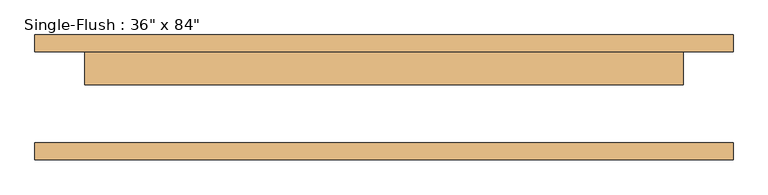
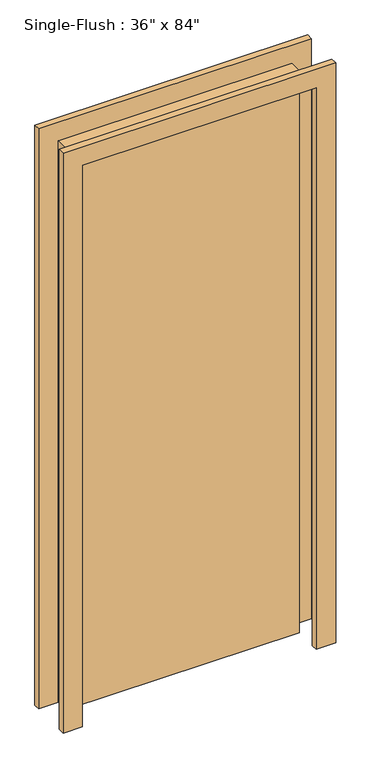
"""IFC4 building model written with IfcOpenShell, lengths in millimetres: door geometry."""

import ifcopenshell
import ifcopenshell.guid

model = None  # the IFC model being written
_history = None  # IfcOwnerHistory: only IFC2X3 demands one
_inside = {}  # id of a spatial element -> (the spatial element, [elements in it])
_under = {}  # id of a project, library or spatial element -> (it, [spatial elements below it])
_declared = {}  # id of a project -> (the project, [libraries it declares])
_typed = {}  # id of a type object -> (the type object, [elements of that type])
_made_of = {}  # id of a material, layer set ... -> (it, [elements and type objects made of it])


def new_model(schema):
    """Start an empty IFC model of exactly this schema.

    Asked for "IFC4X3", IfcOpenShell would pick the latest addendum, in which some entities
    have other attributes; the version numbers below select the first issue.
    IFC2X3 requires an IfcOwnerHistory on every rooted entity: one is made here for all.
    """
    global model, _history
    if schema == "IFC4X3":
        model = ifcopenshell.file(schema_version=(4, 3, 0, 0))
    else:
        model = ifcopenshell.file(schema=schema)
    _inside.clear()
    _under.clear()
    _declared.clear()
    _typed.clear()
    _made_of.clear()
    _history = None
    if model.schema == "IFC2X3":
        org = make("IfcOrganization", Name="unknown")
        user = make(
            "IfcPersonAndOrganization",
            ThePerson=make("IfcPerson", FamilyName="unknown"),
            TheOrganization=org,
        )
        app = make(
            "IfcApplication",
            ApplicationDeveloper=org,
            Version="unknown",
            ApplicationFullName="unknown",
            ApplicationIdentifier="unknown",
        )
        _history = make(
            "IfcOwnerHistory",
            OwningUser=user,
            OwningApplication=app,
            ChangeAction="ADDED",
            CreationDate=0,
        )
    return model


def make(cls, **values):
    """One entity of the class cls with the attributes given. An attribute that is None is left unset."""
    return model.create_entity(
        cls, **{name: value for name, value in values.items() if value is not None}
    )


def rooted(cls, **values):
    """An entity with a GlobalId (a new one), such as an element, a storey or a relation."""
    return make(cls, GlobalId=ifcopenshell.guid.new(), OwnerHistory=_history, **values)


def si_unit(unit_type, name, prefix=None):
    """IfcSIUnit, for example si_unit("LENGTHUNIT", "METRE", prefix="MILLI")."""
    return make("IfcSIUnit", UnitType=unit_type, Prefix=prefix, Name=name)


def assignment(units):
    """IfcUnitAssignment: the units of a project."""
    return None if units is None else make("IfcUnitAssignment", Units=units)


def point(xyz):
    """IfcCartesianPoint."""
    return None if xyz is None else make("IfcCartesianPoint", Coordinates=xyz)


def direction(xyz):
    """IfcDirection."""
    return None if xyz is None else make("IfcDirection", DirectionRatios=xyz)


def frame(location, z_axis=None, x_axis=None):
    """IfcAxis2Placement3D, a coordinate frame: its origin and axes. An axis left out is left unset."""
    return make(
        "IfcAxis2Placement3D",
        Location=point(location),
        Axis=direction(z_axis),
        RefDirection=direction(x_axis),
    )


def origin():
    """The frame at (0, 0, 0) with its axes left unset."""
    return frame((0.0, 0.0, 0.0))


def origin_with_axes():
    """The frame at (0, 0, 0) with the z axis (0, 0, 1) and the x axis (1, 0, 0) written out."""
    return frame((0.0, 0.0, 0.0), z_axis=(0.0, 0.0, 1.0), x_axis=(1.0, 0.0, 0.0))


def place(relative_to, where):
    """IfcLocalPlacement: puts the frame where relative to a parent placement (None: the world)."""
    return make(
        "IfcLocalPlacement", PlacementRelTo=relative_to, RelativePlacement=where
    )


def context(
    kind, dimensions, precision=None, world=None, true_north=None, identifier=None
):
    """IfcGeometricRepresentationContext, for example the 3D "Model" context."""
    return make(
        "IfcGeometricRepresentationContext",
        ContextIdentifier=identifier,
        ContextType=kind,
        CoordinateSpaceDimension=dimensions,
        Precision=precision,
        WorldCoordinateSystem=world,
        TrueNorth=true_north,
    )


def project(units=None, contexts=None):
    """IfcProject with its units and contexts."""
    return rooted(
        "IfcProject",
        Name="project",
        RepresentationContexts=contexts,
        UnitsInContext=assignment(units),
    )


def spatial(cls, under=None, at=None, **own):
    """A site, building, storey or space (cls), placed at a placement, below another one or the project."""
    s = rooted(cls, ObjectPlacement=at, **own)
    if under is not None:
        _under.setdefault(under.id(), (under, []))[1].append(s)
    return s


def polyline(points):
    """IfcPolyline through the points."""
    return make("IfcPolyline", Points=[point(p) for p in points])


def outline(outer, holes=None, kind="AREA"):
    """IfcArbitraryClosedProfileDef: a profile drawn as a closed curve; with holes, ...WithVoids."""
    if holes is None:
        return make("IfcArbitraryClosedProfileDef", ProfileType=kind, OuterCurve=outer)
    return make(
        "IfcArbitraryProfileDefWithVoids",
        ProfileType=kind,
        OuterCurve=outer,
        InnerCurves=holes,
    )


def extrude(swept, where, along, depth):
    """IfcExtrudedAreaSolid: the profile swept, set in the frame where, extruded along a direction by depth."""
    return make(
        "IfcExtrudedAreaSolid",
        SweptArea=swept,
        Position=where,
        ExtrudedDirection=direction(along),
        Depth=depth,
    )


def shape(context_of_items, identifier, shape_type, items):
    """IfcShapeRepresentation: the items that make up one representation, for example the "Body"."""
    return make(
        "IfcShapeRepresentation",
        ContextOfItems=context_of_items,
        RepresentationIdentifier=identifier,
        RepresentationType=shape_type,
        Items=items,
    )


def source(mapping_origin, context_of_items, identifier, shape_type, items):
    """IfcRepresentationMap: a shape defined once, which mapped items show again and again."""
    return make(
        "IfcRepresentationMap",
        MappingOrigin=mapping_origin,
        MappedRepresentation=shape(context_of_items, identifier, shape_type, items),
    )


def transform(
    local_origin,
    x_axis=None,
    y_axis=None,
    z_axis=None,
    scale=None,
    scale2=None,
    scale3=None,
    uniform=True,
):
    """IfcCartesianTransformationOperator3D, or its non-uniform kind. x_axis, y_axis, z_axis: its Axis1, 2, 3."""
    if uniform:
        return make(
            "IfcCartesianTransformationOperator3D",
            Axis1=direction(x_axis),
            Axis2=direction(y_axis),
            LocalOrigin=point(local_origin),
            Scale=scale,
            Axis3=direction(z_axis),
        )
    return make(
        "IfcCartesianTransformationOperator3DnonUniform",
        Axis1=direction(x_axis),
        Axis2=direction(y_axis),
        LocalOrigin=point(local_origin),
        Scale=scale,
        Axis3=direction(z_axis),
        Scale2=scale2,
        Scale3=scale3,
    )


def mapped(mapping_source, mapping_target):
    """IfcMappedItem: shows the shape of a source again, moved by a transform."""
    return make(
        "IfcMappedItem", MappingSource=mapping_source, MappingTarget=mapping_target
    )


def made_of(thing, what):
    """Note that an element or type object is made of a material, layer set ...; save() writes the relation."""
    if what is not None:
        _made_of.setdefault(what.id(), (what, []))[1].append(thing)
    return thing


def element(
    cls,
    number,
    at=None,
    inside=None,
    cuts=None,
    type_object=None,
    material=None,
    context=None,
    identifier="Body",
    shape_type=None,
    held_by="IfcProductDefinitionShape",
    body=None,
    shapes=None,
    **own,
):
    """One element of the class cls, such as IfcWall. Its Tag is "e" and its number.

    at: its placement. inside: the storey or other place that contains it. cuts: it is an
    opening in that element (IfcRelVoidsElement). A single representation is given by context,
    identifier, shape_type and body (its items); several are given by shapes. held_by: the class
    of the entity that holds the representations. save() writes the other relations.
    """
    e = rooted(cls, Tag="e%d" % number, ObjectPlacement=at, **own)
    if body is not None:
        shapes = [shape(context, identifier, shape_type, body)]
    if shapes is not None:
        e.Representation = make(held_by, Representations=shapes)
    if inside is not None:
        _inside.setdefault(inside.id(), (inside, []))[1].append(e)
    if cuts is not None:
        rooted(
            "IfcRelVoidsElement", RelatingBuildingElement=cuts, RelatedOpeningElement=e
        )
    if type_object is not None:
        _typed.setdefault(type_object.id(), (type_object, []))[1].append(e)
    return made_of(e, material)


def aggregate(whole, parts):
    """IfcRelAggregates: a whole, such as a stair, and the parts it consists of."""
    return rooted("IfcRelAggregates", RelatingObject=whole, RelatedObjects=parts)


def save(model, path):
    """Write the relations noted so far, then the file.

    IfcRelAggregates (storeys below a building ...), IfcRelContainedInSpatialStructure (elements
    in a storey), IfcRelDefinesByType, IfcRelAssociatesMaterial and IfcRelDeclares: one each for
    every whole, place, type object, material and project.
    """
    for whole, parts in _under.values():
        aggregate(whole, parts)
    for where, things in _inside.values():
        rooted(
            "IfcRelContainedInSpatialStructure",
            RelatedElements=things,
            RelatingStructure=where,
        )
    for kind, things in _typed.values():
        rooted("IfcRelDefinesByType", RelatedObjects=things, RelatingType=kind)
    for what, things in _made_of.values():
        rooted("IfcRelAssociatesMaterial", RelatedObjects=things, RelatingMaterial=what)
    for by, libraries in _declared.values():
        rooted("IfcRelDeclares", RelatingContext=by, RelatedDefinitions=libraries)
    model.write(path)


def door_de5a2061(model_context):
    return source(origin(), model_context, "Body", "SweptSolid", [
        extrude(outline(polyline([(2399.6, -533.4), (0.0, -533.4), (0.0, -457.2), (2323.4, -457.2), (2323.4, 457.2), (0.0, 457.2), (0.0, 533.4), (2399.6, 533.4), (2399.6, -533.4)])), frame((0.0, 69.85, 0.0), z_axis=(0.0, 1.0, 0.0), x_axis=(0.0, 0.0, 1.0)), (0.0, 0.0, 1.0), 25.4),
        extrude(outline(polyline([(2399.6, 533.4), (2399.6, -533.4), (0.0, -533.4), (0.0, -457.2), (2323.4, -457.2), (2323.4, 457.2), (0.0, 457.2), (0.0, 533.4), (2399.6, 533.4)])), frame((0.0, -95.25, 0.0), z_axis=(0.0, 1.0, 0.0), x_axis=(0.0, 0.0, 1.0)), (0.0, 0.0, 1.0), 25.4),
        extrude(outline(polyline([(457.2, 19.05), (-457.2, 19.05), (-457.2, 69.85), (457.2, 69.85), (457.2, 19.05)])), origin_with_axes(), (0.0, 0.0, 1.0), 2323.4),
    ])


if __name__ == "__main__":
    model = new_model("IFC4")
    model_context = context("Model", 3, world=origin())
    ifc_project = project(units=[si_unit("LENGTHUNIT", "METRE", prefix="MILLI")], contexts=[model_context])
    site = spatial("IfcSite", under=ifc_project)
    building = spatial("IfcBuilding", under=site)
    placement = place(None, origin())
    door_shape = door_de5a2061(model_context)
    element("IfcDoor", 1, ObjectType="Single-Flush : 36\" x 84\"", at=placement, inside=building, context=model_context, shape_type="MappedRepresentation", body=[
        mapped(door_shape, transform((0.0, 0.0, 0.0), x_axis=(1.0, 0.0, 0.0), y_axis=(0.0, 1.0, 0.0), z_axis=(0.0, 0.0, 1.0))),
    ])
    save(model, "model.ifc")

# Revit data of these elements
# Type "Single-Flush : 36\" x 84\""
#   Type Mark = "D2"
#   Construction Type Id = "MDOOR"
#   Assembly Code = "C1020"
#   Analytic Construction = "Metal"
#   Thickness = 50.8 mm
#   Heat Transfer Coefficient (U) = 3.7021 W/(m²·K)
#   Height = 2323.4 mm
#   Trim Projection Ext = 25.4 mm
#   Trim Projection Int = 25.4 mm
#   Trim Width = 76.2 mm
#   Width = 914.4 mm
#   Define Thermal Properties by = 1
#   Door Material = wooden-3
#   Frame Material = wooden-3
#   Visual Light Transmittance = 0
#   Solar Heat Gain Coefficient = 0
#   Function = (empty or 0)
#   Wall Closure = (empty or 0)
# Element 1 (IfcDoor, "Single-Flush : 36\" x 84\"")
#   Materials on its faces: "wooden-3"
# Materials
#   "wooden-3": class "Generic", colour RGB 120 120 120, transparency 0, Cost = 0
